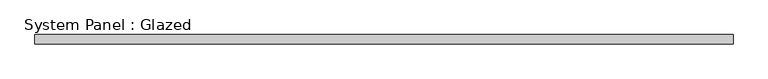
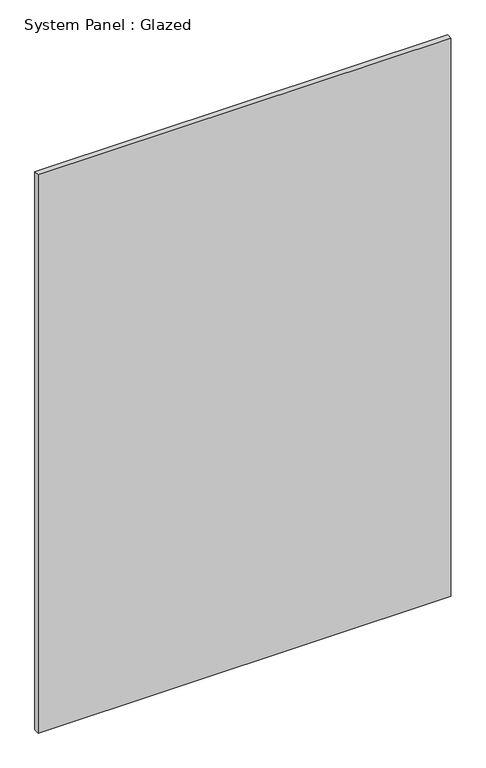
"""IFC4 building model written with IfcOpenShell, lengths in millimetres: plate geometry, System Panel : Glazed."""

from ifc_helpers import new_model, si_unit, origin, origin_with_axes, place, context, project, spatial, polyline, outline, extrude, source, transform, mapped, element, save


def system_panel_glazed_59f98b70(model_context):
    return source(origin(), model_context, "Body", "SweptSolid", [
        extrude(outline(polyline([(918.0833333, 24.5), (-918.0833333, 24.5), (-918.0833333, 49.5), (918.0833333, 49.5), (918.0833333, 24.5)])), origin_with_axes(), (0.0, 0.0, 1.0), 2625.0),
    ])


if __name__ == "__main__":
    model = new_model("IFC4")
    model_context = context("Model", 3, world=origin())
    ifc_project = project(units=[si_unit("LENGTHUNIT", "METRE", prefix="MILLI")], contexts=[model_context])
    site = spatial("IfcSite", under=ifc_project)
    building = spatial("IfcBuilding", under=site)
    placement = place(None, origin())
    system_panel_glazed_shape = system_panel_glazed_59f98b70(model_context)
    element("IfcPlate", 1, ObjectType="System Panel : Glazed", at=placement, inside=building, context=model_context, shape_type="MappedRepresentation", body=[
        mapped(system_panel_glazed_shape, transform((0.0, 0.0, 0.0), x_axis=(1.0, 0.0, 0.0), y_axis=(0.0, 1.0, 0.0), z_axis=(0.0, 0.0, 1.0))),
    ])
    save(model, "model.ifc")

# Revit data of these elements
# Element 1 (IfcPlate, "System Panel : Glazed")
#   Materials on its faces: "Glass"
# Materials
#   "Glass": class "Glass", colour RGB 0 128 192, transparency 0.9
